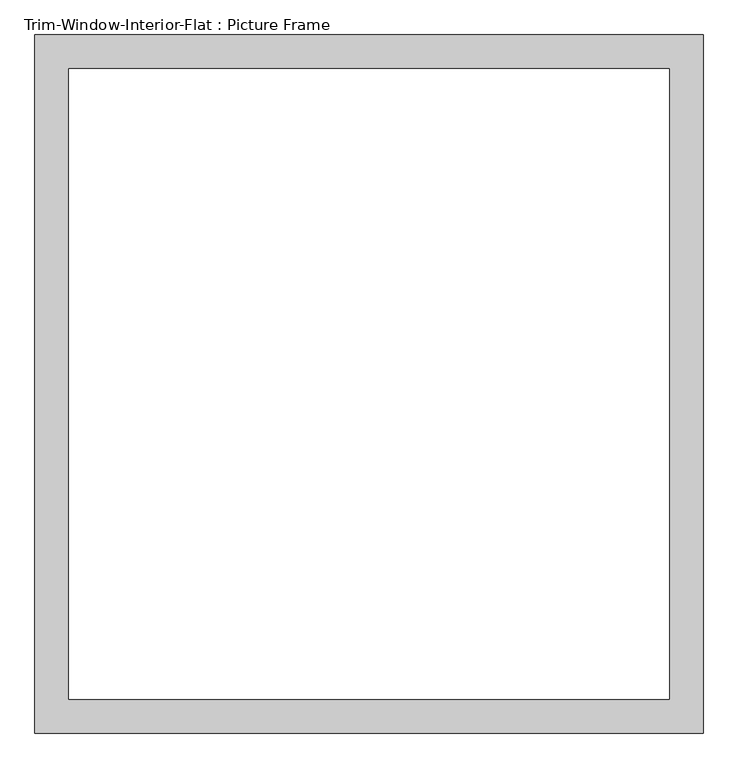
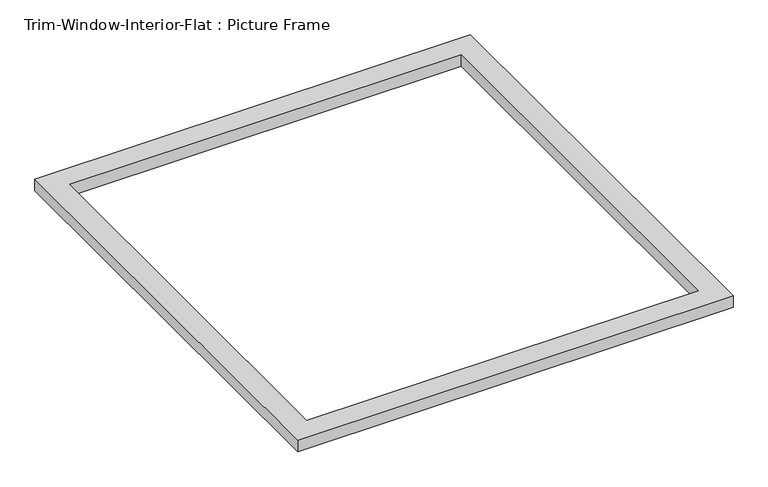
"""IFC4 building model written with IfcOpenShell, lengths in millimetres: proxy geometry, Trim-Window-Interior-Flat : Picture Frame."""

import ifcopenshell
import ifcopenshell.guid

model = None  # the IFC model being written
_history = None  # IfcOwnerHistory: only IFC2X3 demands one
_inside = {}  # id of a spatial element -> (the spatial element, [elements in it])
_under = {}  # id of a project, library or spatial element -> (it, [spatial elements below it])
_declared = {}  # id of a project -> (the project, [libraries it declares])
_typed = {}  # id of a type object -> (the type object, [elements of that type])
_made_of = {}  # id of a material, layer set ... -> (it, [elements and type objects made of it])


def new_model(schema):
    """Start an empty IFC model of exactly this schema.

    Asked for "IFC4X3", IfcOpenShell would pick the latest addendum, in which some entities
    have other attributes; the version numbers below select the first issue.
    IFC2X3 requires an IfcOwnerHistory on every rooted entity: one is made here for all.
    """
    global model, _history
    if schema == "IFC4X3":
        model = ifcopenshell.file(schema_version=(4, 3, 0, 0))
    else:
        model = ifcopenshell.file(schema=schema)
    _inside.clear()
    _under.clear()
    _declared.clear()
    _typed.clear()
    _made_of.clear()
    _history = None
    if model.schema == "IFC2X3":
        org = make("IfcOrganization", Name="unknown")
        user = make(
            "IfcPersonAndOrganization",
            ThePerson=make("IfcPerson", FamilyName="unknown"),
            TheOrganization=org,
        )
        app = make(
            "IfcApplication",
            ApplicationDeveloper=org,
            Version="unknown",
            ApplicationFullName="unknown",
            ApplicationIdentifier="unknown",
        )
        _history = make(
            "IfcOwnerHistory",
            OwningUser=user,
            OwningApplication=app,
            ChangeAction="ADDED",
            CreationDate=0,
        )
    return model


def make(cls, **values):
    """One entity of the class cls with the attributes given. An attribute that is None is left unset."""
    return model.create_entity(
        cls, **{name: value for name, value in values.items() if value is not None}
    )


def rooted(cls, **values):
    """An entity with a GlobalId (a new one), such as an element, a storey or a relation."""
    return make(cls, GlobalId=ifcopenshell.guid.new(), OwnerHistory=_history, **values)


def si_unit(unit_type, name, prefix=None):
    """IfcSIUnit, for example si_unit("LENGTHUNIT", "METRE", prefix="MILLI")."""
    return make("IfcSIUnit", UnitType=unit_type, Prefix=prefix, Name=name)


def assignment(units):
    """IfcUnitAssignment: the units of a project."""
    return None if units is None else make("IfcUnitAssignment", Units=units)


def point(xyz):
    """IfcCartesianPoint."""
    return None if xyz is None else make("IfcCartesianPoint", Coordinates=xyz)


def direction(xyz):
    """IfcDirection."""
    return None if xyz is None else make("IfcDirection", DirectionRatios=xyz)


def frame(location, z_axis=None, x_axis=None):
    """IfcAxis2Placement3D, a coordinate frame: its origin and axes. An axis left out is left unset."""
    return make(
        "IfcAxis2Placement3D",
        Location=point(location),
        Axis=direction(z_axis),
        RefDirection=direction(x_axis),
    )


def origin():
    """The frame at (0, 0, 0) with its axes left unset."""
    return frame((0.0, 0.0, 0.0))


def origin_with_axes():
    """The frame at (0, 0, 0) with the z axis (0, 0, 1) and the x axis (1, 0, 0) written out."""
    return frame((0.0, 0.0, 0.0), z_axis=(0.0, 0.0, 1.0), x_axis=(1.0, 0.0, 0.0))


def place(relative_to, where):
    """IfcLocalPlacement: puts the frame where relative to a parent placement (None: the world)."""
    return make(
        "IfcLocalPlacement", PlacementRelTo=relative_to, RelativePlacement=where
    )


def context(
    kind, dimensions, precision=None, world=None, true_north=None, identifier=None
):
    """IfcGeometricRepresentationContext, for example the 3D "Model" context."""
    return make(
        "IfcGeometricRepresentationContext",
        ContextIdentifier=identifier,
        ContextType=kind,
        CoordinateSpaceDimension=dimensions,
        Precision=precision,
        WorldCoordinateSystem=world,
        TrueNorth=true_north,
    )


def project(units=None, contexts=None):
    """IfcProject with its units and contexts."""
    return rooted(
        "IfcProject",
        Name="project",
        RepresentationContexts=contexts,
        UnitsInContext=assignment(units),
    )


def spatial(cls, under=None, at=None, **own):
    """A site, building, storey or space (cls), placed at a placement, below another one or the project."""
    s = rooted(cls, ObjectPlacement=at, **own)
    if under is not None:
        _under.setdefault(under.id(), (under, []))[1].append(s)
    return s


def polyline(points):
    """IfcPolyline through the points."""
    return make("IfcPolyline", Points=[point(p) for p in points])


def outline(outer, holes=None, kind="AREA"):
    """IfcArbitraryClosedProfileDef: a profile drawn as a closed curve; with holes, ...WithVoids."""
    if holes is None:
        return make("IfcArbitraryClosedProfileDef", ProfileType=kind, OuterCurve=outer)
    return make(
        "IfcArbitraryProfileDefWithVoids",
        ProfileType=kind,
        OuterCurve=outer,
        InnerCurves=holes,
    )


def extrude(swept, where, along, depth):
    """IfcExtrudedAreaSolid: the profile swept, set in the frame where, extruded along a direction by depth."""
    return make(
        "IfcExtrudedAreaSolid",
        SweptArea=swept,
        Position=where,
        ExtrudedDirection=direction(along),
        Depth=depth,
    )


def shape(context_of_items, identifier, shape_type, items):
    """IfcShapeRepresentation: the items that make up one representation, for example the "Body"."""
    return make(
        "IfcShapeRepresentation",
        ContextOfItems=context_of_items,
        RepresentationIdentifier=identifier,
        RepresentationType=shape_type,
        Items=items,
    )


def source(mapping_origin, context_of_items, identifier, shape_type, items):
    """IfcRepresentationMap: a shape defined once, which mapped items show again and again."""
    return make(
        "IfcRepresentationMap",
        MappingOrigin=mapping_origin,
        MappedRepresentation=shape(context_of_items, identifier, shape_type, items),
    )


def transform(
    local_origin,
    x_axis=None,
    y_axis=None,
    z_axis=None,
    scale=None,
    scale2=None,
    scale3=None,
    uniform=True,
):
    """IfcCartesianTransformationOperator3D, or its non-uniform kind. x_axis, y_axis, z_axis: its Axis1, 2, 3."""
    if uniform:
        return make(
            "IfcCartesianTransformationOperator3D",
            Axis1=direction(x_axis),
            Axis2=direction(y_axis),
            LocalOrigin=point(local_origin),
            Scale=scale,
            Axis3=direction(z_axis),
        )
    return make(
        "IfcCartesianTransformationOperator3DnonUniform",
        Axis1=direction(x_axis),
        Axis2=direction(y_axis),
        LocalOrigin=point(local_origin),
        Scale=scale,
        Axis3=direction(z_axis),
        Scale2=scale2,
        Scale3=scale3,
    )


def mapped(mapping_source, mapping_target):
    """IfcMappedItem: shows the shape of a source again, moved by a transform."""
    return make(
        "IfcMappedItem", MappingSource=mapping_source, MappingTarget=mapping_target
    )


def made_of(thing, what):
    """Note that an element or type object is made of a material, layer set ...; save() writes the relation."""
    if what is not None:
        _made_of.setdefault(what.id(), (what, []))[1].append(thing)
    return thing


def element(
    cls,
    number,
    at=None,
    inside=None,
    cuts=None,
    type_object=None,
    material=None,
    context=None,
    identifier="Body",
    shape_type=None,
    held_by="IfcProductDefinitionShape",
    body=None,
    shapes=None,
    **own,
):
    """One element of the class cls, such as IfcWall. Its Tag is "e" and its number.

    at: its placement. inside: the storey or other place that contains it. cuts: it is an
    opening in that element (IfcRelVoidsElement). A single representation is given by context,
    identifier, shape_type and body (its items); several are given by shapes. held_by: the class
    of the entity that holds the representations. save() writes the other relations.
    """
    e = rooted(cls, Tag="e%d" % number, ObjectPlacement=at, **own)
    if body is not None:
        shapes = [shape(context, identifier, shape_type, body)]
    if shapes is not None:
        e.Representation = make(held_by, Representations=shapes)
    if inside is not None:
        _inside.setdefault(inside.id(), (inside, []))[1].append(e)
    if cuts is not None:
        rooted(
            "IfcRelVoidsElement", RelatingBuildingElement=cuts, RelatedOpeningElement=e
        )
    if type_object is not None:
        _typed.setdefault(type_object.id(), (type_object, []))[1].append(e)
    return made_of(e, material)


def aggregate(whole, parts):
    """IfcRelAggregates: a whole, such as a stair, and the parts it consists of."""
    return rooted("IfcRelAggregates", RelatingObject=whole, RelatedObjects=parts)


def save(model, path):
    """Write the relations noted so far, then the file.

    IfcRelAggregates (storeys below a building ...), IfcRelContainedInSpatialStructure (elements
    in a storey), IfcRelDefinesByType, IfcRelAssociatesMaterial and IfcRelDeclares: one each for
    every whole, place, type object, material and project.
    """
    for whole, parts in _under.values():
        aggregate(whole, parts)
    for where, things in _inside.values():
        rooted(
            "IfcRelContainedInSpatialStructure",
            RelatedElements=things,
            RelatingStructure=where,
        )
    for kind, things in _typed.values():
        rooted("IfcRelDefinesByType", RelatedObjects=things, RelatingType=kind)
    for what, things in _made_of.values():
        rooted("IfcRelAssociatesMaterial", RelatedObjects=things, RelatingMaterial=what)
    for by, libraries in _declared.values():
        rooted("IfcRelDeclares", RelatingContext=by, RelatedDefinitions=libraries)
    model.write(path)


def trim_window_interior_flat_picture_frame_be940afe(model_context):
    return source(origin(), model_context, "Body", "SweptSolid", [
        extrude(outline(polyline([(565.15, 44.45), (565.15, -1136.65), (-565.15, -1136.65), (-565.15, 44.45), (565.15, 44.45)]), holes=[polyline([(508.0, -12.7), (-508.0, -12.7), (-508.0, -1079.5), (508.0, -1079.5), (508.0, -12.7)])]), origin_with_axes(), (0.0, 0.0, 1.0), 31.75),
    ])


if __name__ == "__main__":
    model = new_model("IFC4")
    model_context = context("Model", 3, world=origin())
    ifc_project = project(units=[si_unit("LENGTHUNIT", "METRE", prefix="MILLI")], contexts=[model_context])
    site = spatial("IfcSite", under=ifc_project)
    building = spatial("IfcBuilding", under=site)
    placement = place(None, origin())
    trim_window_interior_flat_picture_frame_shape = trim_window_interior_flat_picture_frame_be940afe(model_context)
    element("IfcBuildingElementProxy", 1, Name="Trim-Window-Interior-Flat : Picture Frame", ObjectType="Trim-Window-Interior-Flat : Picture Frame", at=placement, inside=building, context=model_context, shape_type="MappedRepresentation", body=[
        mapped(trim_window_interior_flat_picture_frame_shape, transform((0.0, 0.0, 0.0), x_axis=(1.0, 0.0, 0.0), y_axis=(0.0, 1.0, 0.0), z_axis=(0.0, 0.0, 1.0))),
    ])
    save(model, "model.ifc")

# Revit data of these elements
# Type "Trim-Window-Interior-Flat : Picture Frame"
#   Trim Thickness_Picture Frame = 0' - 1 1/4"
#   Trim Width = 0' - 2 1/4"
#   Trim Thickness_with Sill = 0' - 0 3/4"
#   Sill Thickness = 0' - 1 1/4"
#   Opening Width [instance default] = 2' - 0"
#   Opening Height [instance default] = 3' - 0"
#   Default Elevation = 4' - 0"
#   Sill = no
#   Picture Frame = yes
#   Trim Material [instance default] = none
# Element 1 (IfcBuildingElementProxy, "Trim-Window-Interior-Flat : Picture Frame")
#   Opening Width = 3' - 5"
#   Opening Height = 3' - 7"
#   Trim Material = Wood - Stained
#   Materials on its faces: "Wood - Stained"
# Materials
#   "Wood - Stained": class "Wood", colour RGB 224 178 126, transparency 0, Cost = 0
